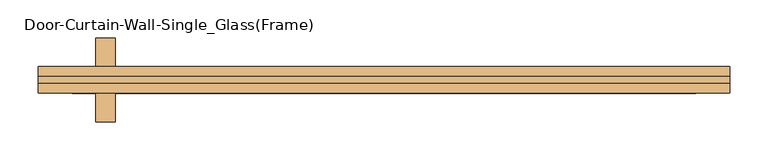
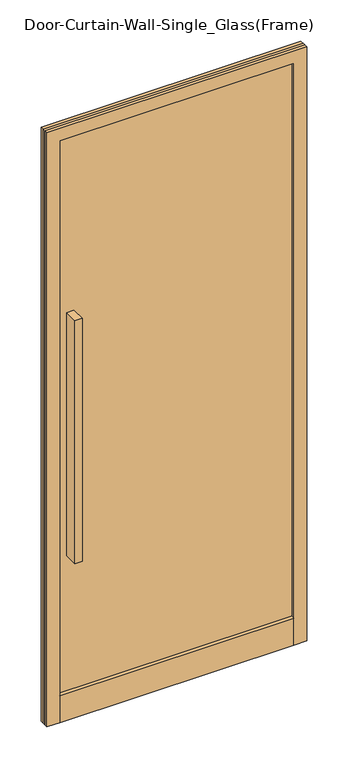
"""IFC4 building model written with IfcOpenShell, lengths in millimetres: door geometry, Door-Curtain-Wall-Single_Glass(Frame) : H_DR_AR B12_Door_Single_Glass_W1000xH2200_SSD-1."""

from ifc_helpers import new_model, si_unit, frame, origin, origin_with_axes, place, context, project, spatial, polyline, outline, extrude, source, transform, mapped, element, save


def door_curtain_wall_single_glass_frame_6d520873(model_context):
    return source(origin(), model_context, "Body", "SweptSolid", [
        extrude(outline(polyline([(455.0, 0.0), (455.0, -9.0), (-455.0, -9.0), (-455.0, 0.0), (455.0, 0.0)])), origin_with_axes(), (0.0, 0.0, 1.0), 2200.0),
        extrude(outline(polyline([(-353.4, 50.8), (-353.4, 0.0), (-378.8, 0.0), (-378.8, 50.8), (-353.4, 50.8)])), frame((0.0, 0.0, 600.0), z_axis=(0.0, 0.0, 1.0), x_axis=(1.0, 0.0, 0.0)), (0.0, 0.0, 1.0), 900.0),
        extrude(outline(polyline([(-378.8, -59.8), (-378.8, -9.0), (-353.4, -9.0), (-353.4, -59.8), (-378.8, -59.8)])), frame((0.0, 0.0, 600.0), z_axis=(0.0, 0.0, 1.0), x_axis=(1.0, 0.0, 0.0)), (0.0, 0.0, 1.0), 900.0),
        extrude(outline(polyline([(0.0, 455.0), (2200.0, 455.0), (2200.0, -455.0), (0.0, -455.0), (0.0, -410.0), (2155.0, -410.0), (2155.0, 410.0), (0.0, 410.0), (0.0, 455.0)])), frame((0.0, -22.0, 0.0), z_axis=(0.0, 1.0, 0.0), x_axis=(0.0, 0.0, 1.0)), (0.0, 0.0, 1.0), 35.0),
        extrude(outline(polyline([(410.0, -22.0), (-410.0, -22.0), (-410.0, 13.0), (410.0, 13.0), (410.0, -22.0)])), origin_with_axes(), (0.0, 0.0, 1.0), 100.0),
    ])


if __name__ == "__main__":
    model = new_model("IFC4")
    model_context = context("Model", 3, world=origin())
    ifc_project = project(units=[si_unit("LENGTHUNIT", "METRE", prefix="MILLI")], contexts=[model_context])
    site = spatial("IfcSite", under=ifc_project)
    building = spatial("IfcBuilding", under=site)
    placement = place(None, origin())
    door_curtain_wall_single_glass_frame_shape = door_curtain_wall_single_glass_frame_6d520873(model_context)
    element("IfcDoor", 1, ObjectType="Door-Curtain-Wall-Single_Glass(Frame) : H_DR_AR B12_Door_Single_Glass_W1000xH2200_SSD-1", at=placement, inside=building, context=model_context, shape_type="MappedRepresentation", body=[
        mapped(door_curtain_wall_single_glass_frame_shape, transform((0.0, 0.0, 0.0), x_axis=(1.0, 0.0, 0.0), y_axis=(0.0, 1.0, 0.0), z_axis=(0.0, 0.0, 1.0))),
    ])
    save(model, "model.ifc")

# Revit data of these elements
# Type "Door-Curtain-Wall-Single_Glass(Frame) : H_DR_AR B12_Door_Single_Glass_W1000xH2200_SSD-1"
#   Type Mark = "448"
#   Assembly Code = "B2030100"
#   Analytic Construction = "<None>"
#   Width [instance default] = 914.4 mm
#   Thermal Resistance (R) = 1.7611 (m²·K)/W
#   Swing Angle [instance default] = 90.00°
#   Frame Thk. = 45 mm
#   Frame_Thk2 = 100 mm
#   Heat Transfer Coefficient (U) = 0.567826 W/(m²·K)
#   Offset = 0 mm
#   Define Thermal Properties by = 1
#   Door Handle Material = 00_Metal_Stainless Steel
#   Glazing = 00_F_Glass
#   Visual Light Transmittance = 0
#   Solar Heat Gain Coefficient = 0
#   Construction Type Id = ""
#   Function = (empty or 0)
# Element 1 (IfcDoor, "Door-Curtain-Wall-Single_Glass(Frame) : H_DR_AR B12_Door_Single_Glass_W1000xH2200_SSD-1")
#   Width = 910 mm
#   Materials on its faces: "00_Metal_Stainless Steel", "00_F_Glass"
# Materials
#   "00_Metal_Stainless Steel": class "Metal", colour RGB 148 148 148, transparency 0, Description = "Steel", Cost = 0
#   "00_F_Glass": class "Glass", colour RGB 218 227 224, transparency 0.85, Description = "Glass", Cost = 0
